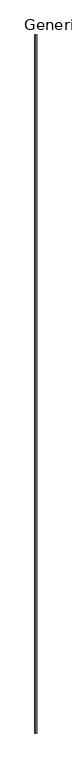
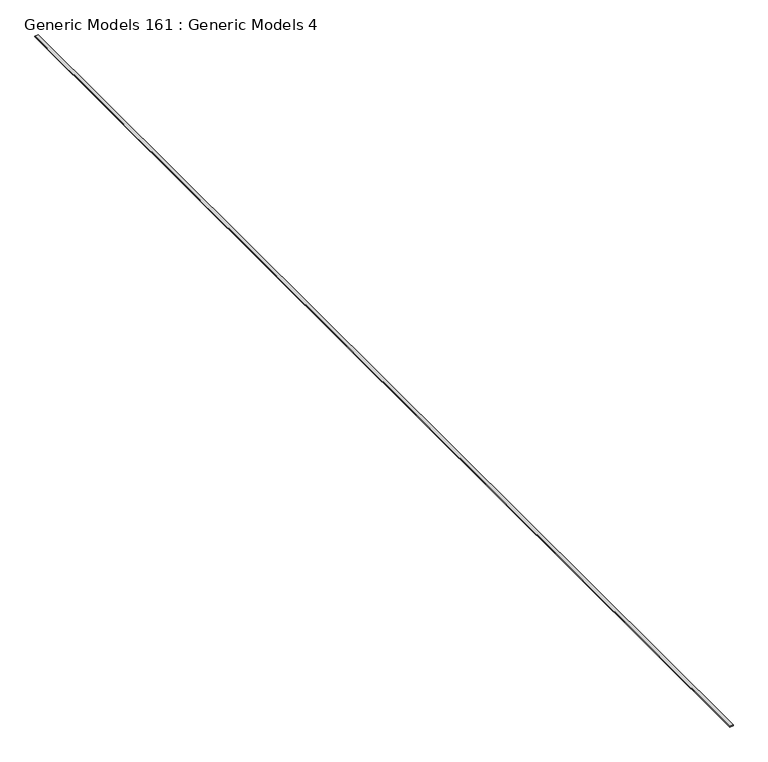
"""IFC4 building model written with IfcOpenShell, lengths in millimetres: proxy geometry, Generic Models 161 : Generic Models 4."""

from ifc_helpers import new_model, si_unit, point, frame, frame_2d, origin, place, context, project, spatial, polyline, circle_curve, trimmed, segment, composite_curve, outline, extrude, source, transform, mapped, element, save


def generic_models_161_generic_models_4_e7cb0811(model_context):
    return source(origin(), model_context, "Body", "SweptSolid", [
        extrude(outline(composite_curve([segment(trimmed(circle_curve(frame_2d((122958.8234874, -10292.4988366)), 5.3394144), [point((122963.5859874, -10290.0847239))], [point((122954.0609874, -10290.0847239))], True, "CARTESIAN"), True, "CONTINUOUS"), segment(polyline([(122954.0609874, -10290.0847239), (122954.0609874, -10252.9339552), (122963.5859874, -10252.9339552), (122963.5859874, -10290.0847239)]), True, "CONTINUOUS")], self_intersect=False)), frame((0.0, -5493.3230338, 0.0), z_axis=(0.0, 1.0, 0.0), x_axis=(0.0, 0.0, 1.0)), (0.0, 0.0, 1.0), 12547.6),
    ])


if __name__ == "__main__":
    model = new_model("IFC4")
    model_context = context("Model", 3, world=origin())
    ifc_project = project(units=[si_unit("LENGTHUNIT", "METRE", prefix="MILLI")], contexts=[model_context])
    site = spatial("IfcSite", under=ifc_project)
    building = spatial("IfcBuilding", under=site)
    placement = place(None, origin())
    generic_models_161_generic_models_4_shape = generic_models_161_generic_models_4_e7cb0811(model_context)
    element("IfcBuildingElementProxy", 1, Name="Generic Models 161 : Generic Models 4", ObjectType="Generic Models 161 : Generic Models 4", at=placement, inside=building, context=model_context, shape_type="MappedRepresentation", body=[
        mapped(generic_models_161_generic_models_4_shape, transform((0.0, 0.0, 0.0), x_axis=(1.0, 0.0, 0.0), y_axis=(0.0, 1.0, 0.0), z_axis=(0.0, 0.0, 1.0))),
    ])
    save(model, "model.ifc")

# Revit data of these elements
# Element 1 (IfcBuildingElementProxy, "Generic Models 161 : Generic Models 4")
#   Materials on its faces: "_MORTAR SETTING BED"
# Materials
#   "_MORTAR SETTING BED": class "Generic", colour RGB 191 191 191, transparency 0, Cost = 0
